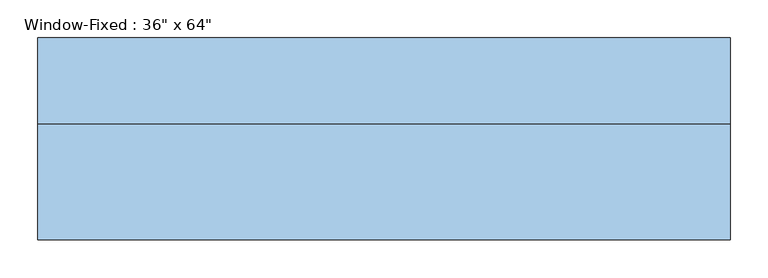
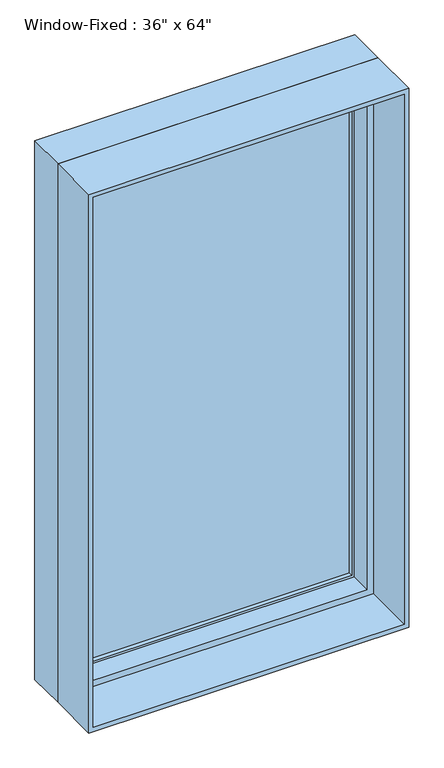
"""IFC4 building model written with IfcOpenShell, lengths in millimetres: window geometry."""

from ifc_helpers import new_model, si_unit, frame, origin, place, context, project, spatial, polyline, outline, extrude, faceted_brep, source, transform, mapped, element, save


def window_886270d0(model_context):
    return source(origin(), model_context, "Body", "SolidModel", [
        extrude(outline(polyline([(419.1, 79.375), (419.1, 73.025), (-419.1, 73.025), (-419.1, 79.375), (419.1, 79.375)])), frame((0.0, 0.0, 952.5), z_axis=(0.0, 0.0, 1.0), x_axis=(1.0, 0.0, 0.0)), (0.0, 0.0, 1.0), 1549.4),
        extrude(outline(polyline([(-419.1, 60.325), (-419.1, 66.675), (419.1, 66.675), (419.1, 60.325), (-419.1, 60.325)])), frame((0.0, 0.0, 952.5), z_axis=(0.0, 0.0, 1.0), x_axis=(1.0, 0.0, 0.0)), (0.0, 0.0, 1.0), 1549.4),
        extrude(outline(polyline([(927.1, 444.5), (2527.3, 444.5), (2527.3, -444.5), (927.1, -444.5), (927.1, 444.5)]), holes=[polyline([(952.5, -419.1), (2501.9, -419.1), (2501.9, 419.1), (952.5, 419.1), (952.5, -419.1)])]), frame((0.0, 47.625, 0.0), z_axis=(0.0, 1.0, 0.0), x_axis=(0.0, 0.0, 1.0)), (0.0, 0.0, 1.0), 44.45),
        extrude(outline(polyline([(2540.0, -457.2), (914.4, -457.2), (914.4, 457.2), (2540.0, 457.2), (2540.0, -457.2)]), holes=[polyline([(2527.3, 444.5), (927.1, 444.5), (927.1, -444.5), (2527.3, -444.5), (2527.3, 444.5)])]), frame((0.0, -168.275, 0.0), z_axis=(0.0, 1.0, 0.0), x_axis=(0.0, 0.0, 1.0)), (0.0, 0.0, 1.0), 152.4),
        faceted_brep([(457.2, -15.875, 2540.0), (457.2, 98.425, 2540.0), (-457.2, 98.425, 2540.0), (-457.2, -15.875, 2540.0), (-457.2, 98.425, 914.4), (-457.2, -15.875, 914.4), (457.2, 98.425, 914.4), (457.2, -15.875, 914.4), (425.45, -15.875, 2508.25), (425.45, -15.875, 946.15), (-425.45, -15.875, 946.15), (-425.45, -15.875, 2508.25), (-444.5, 98.425, 2527.3), (-444.5, 98.425, 927.1), (444.5, 98.425, 927.1), (444.5, 98.425, 2527.3), (425.45, 47.625, 2508.25), (-425.45, 47.625, 2508.25), (444.5, 47.625, 2527.3), (-444.5, 47.625, 2527.3), (-425.45, 47.625, 946.15), (-444.5, 47.625, 927.1), (425.45, 47.625, 946.15), (444.5, 47.625, 927.1)], [[[0, 1, 2, 3]], [[3, 2, 4, 5]], [[5, 4, 6, 7]], [[3, 5, 7, 0], [8, 9, 10, 11]], [[7, 6, 1, 0]], [[1, 6, 4, 2], [12, 13, 14, 15]], [[16, 8, 11, 17]], [[15, 18, 19, 12]], [[17, 11, 10, 20]], [[12, 19, 21, 13]], [[20, 10, 9, 22]], [[13, 21, 23, 14]], [[22, 9, 8, 16]], [[18, 23, 21, 19], [17, 20, 22, 16]], [[14, 23, 18, 15]]]),
    ])


if __name__ == "__main__":
    model = new_model("IFC4")
    model_context = context("Model", 3, world=origin())
    ifc_project = project(units=[si_unit("LENGTHUNIT", "METRE", prefix="MILLI")], contexts=[model_context])
    site = spatial("IfcSite", under=ifc_project)
    building = spatial("IfcBuilding", under=site)
    placement = place(None, origin())
    window_shape = window_886270d0(model_context)
    element("IfcWindow", 1, ObjectType="Window-Fixed : 36\" x 64\"", at=placement, inside=building, context=model_context, shape_type="MappedRepresentation", body=[
        mapped(window_shape, transform((0.0, 0.0, 0.0), x_axis=(1.0, 0.0, 0.0), y_axis=(0.0, 1.0, 0.0), z_axis=(0.0, 0.0, 1.0))),
    ])
    save(model, "model.ifc")

# Revit data of these elements
# Type "Window-Fixed : 36\" x 64\""
#   Type Mark = "23"
#   Fire Rating = "0.5h"
#   Assembly Code = "B2020100"
#   Analytic Construction = "Double glazing - domestic"
#   Window Inset [instance default] = 0' - 0"
#   Wall Thickness [instance default] = 0' - 6"
#   Visual Light Transmittance = 0.81
#   Thermal Resistance (R) = 1.8146 (h·ft²·°F)/BTU
#   Solar Heat Gain Coefficient = 0.76
#   Rough Width = 3' - 0 1/2"
#   Rough Height = 5' - 4 1/2"
#   Interior Wall Closure [instance default] = 0' - 2 1/4"
#   Height = 5' - 4"
#   Heat Transfer Coefficient (U) = 0.5511 BTU/(h·ft²·°F)
#   Frame Extension [instance default] = 0' - 0 1/4"
#   Exterior Wall Closure [instance default] = 0' - 1 1/4"
#   Extension Jamb [instance default] = 0' - 2 1/4"
#   Default Sill Height = 3' - 0"
#   Width = 3' - 0"
#   Muntin Visibility = yes
#   Interior Trim Visibility [instance default] = yes
#   Exterior Trim Visibility [instance default] = yes
#   Extension Jamb Visibility [instance default] = yes
#   Muntin Pattern = Muntin Pattern_2x2 : Muntin Pattern_2x2
#   Interior Trim Material = Wood - Stained
#   Interior Trim = Trim-Window-Interior-Flat : Picture Frame
#   Interior Frame Material = Wood - Stained
#   Glass Panel Material = Glass
#   Exterior Trim Material = Clad - White
#   Exterior Trim = Trim-Window-Exterior-Flat : with Sill
#   Exterior Frame Material = Clad - White
#   Wall Closure = (empty or 0)
# Element 1 (IfcWindow, "Window-Fixed : 36\" x 64\"")
#   Window Inset = 0' - 3 1/2"
#   Wall Thickness = 1' - 1 1/4"
#   Exterior Wall Closure = 0' - 5 1/2"
#   Extension Jamb = 0' - 6"
#   Exterior Trim Visibility = no
#   Materials on its faces: "Wood - Stained", "Glass", "Clad - White"
# Materials
#   "Wood - Stained": class "Wood", colour RGB 224 178 126, transparency 0, Cost = 0
#   "Glass": class "Glass", colour RGB 0 128 192, transparency 0.75, Description = "Soda Lime Glass", Cost = 0
#   "Clad - White": class "Wood", colour RGB 242 242 238, transparency 0, Cost = 0
